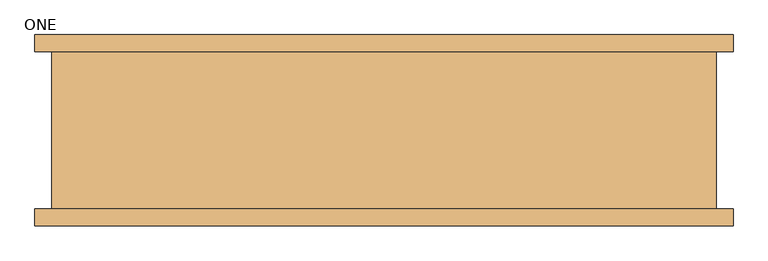
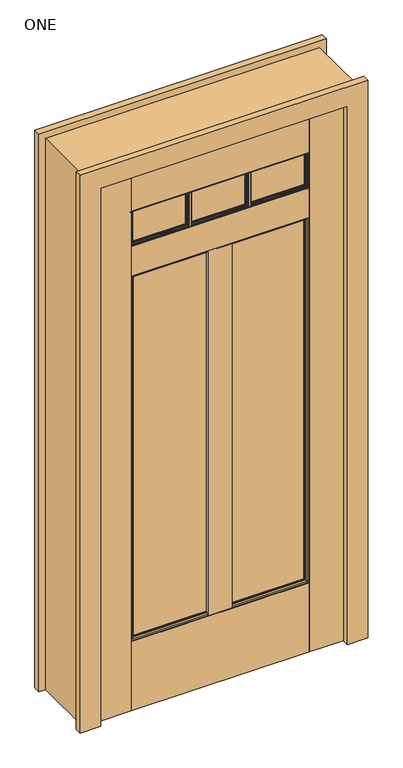
"""IFC4 building model written with IfcOpenShell, lengths in millimetres: door geometry, Door-Exterior-Simpson-Craftsman : ONE."""

import ifcopenshell
import ifcopenshell.guid

model = None  # the IFC model being written
_history = None  # IfcOwnerHistory: only IFC2X3 demands one
_inside = {}  # id of a spatial element -> (the spatial element, [elements in it])
_under = {}  # id of a project, library or spatial element -> (it, [spatial elements below it])
_declared = {}  # id of a project -> (the project, [libraries it declares])
_typed = {}  # id of a type object -> (the type object, [elements of that type])
_made_of = {}  # id of a material, layer set ... -> (it, [elements and type objects made of it])


def new_model(schema):
    """Start an empty IFC model of exactly this schema.

    Asked for "IFC4X3", IfcOpenShell would pick the latest addendum, in which some entities
    have other attributes; the version numbers below select the first issue.
    IFC2X3 requires an IfcOwnerHistory on every rooted entity: one is made here for all.
    """
    global model, _history
    if schema == "IFC4X3":
        model = ifcopenshell.file(schema_version=(4, 3, 0, 0))
    else:
        model = ifcopenshell.file(schema=schema)
    _inside.clear()
    _under.clear()
    _declared.clear()
    _typed.clear()
    _made_of.clear()
    _history = None
    if model.schema == "IFC2X3":
        org = make("IfcOrganization", Name="unknown")
        user = make(
            "IfcPersonAndOrganization",
            ThePerson=make("IfcPerson", FamilyName="unknown"),
            TheOrganization=org,
        )
        app = make(
            "IfcApplication",
            ApplicationDeveloper=org,
            Version="unknown",
            ApplicationFullName="unknown",
            ApplicationIdentifier="unknown",
        )
        _history = make(
            "IfcOwnerHistory",
            OwningUser=user,
            OwningApplication=app,
            ChangeAction="ADDED",
            CreationDate=0,
        )
    return model


def make(cls, **values):
    """One entity of the class cls with the attributes given. An attribute that is None is left unset."""
    return model.create_entity(
        cls, **{name: value for name, value in values.items() if value is not None}
    )


def rooted(cls, **values):
    """An entity with a GlobalId (a new one), such as an element, a storey or a relation."""
    return make(cls, GlobalId=ifcopenshell.guid.new(), OwnerHistory=_history, **values)


def si_unit(unit_type, name, prefix=None):
    """IfcSIUnit, for example si_unit("LENGTHUNIT", "METRE", prefix="MILLI")."""
    return make("IfcSIUnit", UnitType=unit_type, Prefix=prefix, Name=name)


def assignment(units):
    """IfcUnitAssignment: the units of a project."""
    return None if units is None else make("IfcUnitAssignment", Units=units)


def point(xyz):
    """IfcCartesianPoint."""
    return None if xyz is None else make("IfcCartesianPoint", Coordinates=xyz)


def direction(xyz):
    """IfcDirection."""
    return None if xyz is None else make("IfcDirection", DirectionRatios=xyz)


def frame(location, z_axis=None, x_axis=None):
    """IfcAxis2Placement3D, a coordinate frame: its origin and axes. An axis left out is left unset."""
    return make(
        "IfcAxis2Placement3D",
        Location=point(location),
        Axis=direction(z_axis),
        RefDirection=direction(x_axis),
    )


def frame_2d(location, x_axis=None):
    """IfcAxis2Placement2D, a coordinate frame in the plane: its origin and x axis."""
    return make(
        "IfcAxis2Placement2D", Location=point(location), RefDirection=direction(x_axis)
    )


def origin():
    """The frame at (0, 0, 0) with its axes left unset."""
    return frame((0.0, 0.0, 0.0))


def origin_with_axes():
    """The frame at (0, 0, 0) with the z axis (0, 0, 1) and the x axis (1, 0, 0) written out."""
    return frame((0.0, 0.0, 0.0), z_axis=(0.0, 0.0, 1.0), x_axis=(1.0, 0.0, 0.0))


def place(relative_to, where):
    """IfcLocalPlacement: puts the frame where relative to a parent placement (None: the world)."""
    return make(
        "IfcLocalPlacement", PlacementRelTo=relative_to, RelativePlacement=where
    )


def context(
    kind, dimensions, precision=None, world=None, true_north=None, identifier=None
):
    """IfcGeometricRepresentationContext, for example the 3D "Model" context."""
    return make(
        "IfcGeometricRepresentationContext",
        ContextIdentifier=identifier,
        ContextType=kind,
        CoordinateSpaceDimension=dimensions,
        Precision=precision,
        WorldCoordinateSystem=world,
        TrueNorth=true_north,
    )


def project(units=None, contexts=None):
    """IfcProject with its units and contexts."""
    return rooted(
        "IfcProject",
        Name="project",
        RepresentationContexts=contexts,
        UnitsInContext=assignment(units),
    )


def spatial(cls, under=None, at=None, **own):
    """A site, building, storey or space (cls), placed at a placement, below another one or the project."""
    s = rooted(cls, ObjectPlacement=at, **own)
    if under is not None:
        _under.setdefault(under.id(), (under, []))[1].append(s)
    return s


def polyline(points):
    """IfcPolyline through the points."""
    return make("IfcPolyline", Points=[point(p) for p in points])


def circle_curve(where, radius):
    """IfcCircle in the frame where."""
    return make("IfcCircle", Position=where, Radius=radius)


def ellipse_curve(where, semi_axis1, semi_axis2):
    """IfcEllipse in the frame where."""
    return make(
        "IfcEllipse", Position=where, SemiAxis1=semi_axis1, SemiAxis2=semi_axis2
    )


def trimmed(basis, trim1, trim2, sense, master):
    """IfcTrimmedCurve: the piece of a basis curve between two trims."""
    return make(
        "IfcTrimmedCurve",
        BasisCurve=basis,
        Trim1=trim1,
        Trim2=trim2,
        SenseAgreement=sense,
        MasterRepresentation=master,
    )


def segment(curve, same_sense, transition):
    """IfcCompositeCurveSegment."""
    return make(
        "IfcCompositeCurveSegment",
        Transition=transition,
        SameSense=same_sense,
        ParentCurve=curve,
    )


def composite_curve(segments, self_intersect=None):
    """IfcCompositeCurve: segments joined end to end."""
    return make("IfcCompositeCurve", Segments=segments, SelfIntersect=self_intersect)


def outline(outer, holes=None, kind="AREA"):
    """IfcArbitraryClosedProfileDef: a profile drawn as a closed curve; with holes, ...WithVoids."""
    if holes is None:
        return make("IfcArbitraryClosedProfileDef", ProfileType=kind, OuterCurve=outer)
    return make(
        "IfcArbitraryProfileDefWithVoids",
        ProfileType=kind,
        OuterCurve=outer,
        InnerCurves=holes,
    )


def extrude(swept, where, along, depth):
    """IfcExtrudedAreaSolid: the profile swept, set in the frame where, extruded along a direction by depth."""
    return make(
        "IfcExtrudedAreaSolid",
        SweptArea=swept,
        Position=where,
        ExtrudedDirection=direction(along),
        Depth=depth,
    )


def faces_of(points, faces, orient=None, outer=None):
    """IfcFace entities. A face is a list of loops; a loop is a list of indices into points, from 0.

    orient and outer hold one flag for each loop. By default every Orientation is true, the
    first loop of a face is its IfcFaceOuterBound and the others are IfcFaceBound.
    """
    made = []
    for i, loops in enumerate(faces):
        bounds = []
        for j, loop in enumerate(loops):
            is_outer = j == 0 if outer is None else outer[i][j]
            bounds.append(
                make(
                    "IfcFaceOuterBound" if is_outer else "IfcFaceBound",
                    Bound=make("IfcPolyLoop", Polygon=[points[k] for k in loop]),
                    Orientation=True if orient is None else orient[i][j],
                )
            )
        made.append(make("IfcFace", Bounds=bounds))
    return made


def faceted_brep(points, faces, orient=None, outer=None, voids=None):
    """IfcFacetedBrep: a solid bounded by flat faces; with voids (closed shells), ...WithVoids."""
    shared = [point(p) for p in points]
    hull = make("IfcClosedShell", CfsFaces=faces_of(shared, faces, orient, outer))
    if voids is None:
        return make("IfcFacetedBrep", Outer=hull)
    return make(
        "IfcFacetedBrepWithVoids",
        Outer=hull,
        Voids=[
            make(cls, CfsFaces=faces_of(shared, fs, o, b)) for cls, fs, o, b in voids
        ],
    )


def shape(context_of_items, identifier, shape_type, items):
    """IfcShapeRepresentation: the items that make up one representation, for example the "Body"."""
    return make(
        "IfcShapeRepresentation",
        ContextOfItems=context_of_items,
        RepresentationIdentifier=identifier,
        RepresentationType=shape_type,
        Items=items,
    )


def source(mapping_origin, context_of_items, identifier, shape_type, items):
    """IfcRepresentationMap: a shape defined once, which mapped items show again and again."""
    return make(
        "IfcRepresentationMap",
        MappingOrigin=mapping_origin,
        MappedRepresentation=shape(context_of_items, identifier, shape_type, items),
    )


def transform(
    local_origin,
    x_axis=None,
    y_axis=None,
    z_axis=None,
    scale=None,
    scale2=None,
    scale3=None,
    uniform=True,
):
    """IfcCartesianTransformationOperator3D, or its non-uniform kind. x_axis, y_axis, z_axis: its Axis1, 2, 3."""
    if uniform:
        return make(
            "IfcCartesianTransformationOperator3D",
            Axis1=direction(x_axis),
            Axis2=direction(y_axis),
            LocalOrigin=point(local_origin),
            Scale=scale,
            Axis3=direction(z_axis),
        )
    return make(
        "IfcCartesianTransformationOperator3DnonUniform",
        Axis1=direction(x_axis),
        Axis2=direction(y_axis),
        LocalOrigin=point(local_origin),
        Scale=scale,
        Axis3=direction(z_axis),
        Scale2=scale2,
        Scale3=scale3,
    )


def mapped(mapping_source, mapping_target):
    """IfcMappedItem: shows the shape of a source again, moved by a transform."""
    return make(
        "IfcMappedItem", MappingSource=mapping_source, MappingTarget=mapping_target
    )


def made_of(thing, what):
    """Note that an element or type object is made of a material, layer set ...; save() writes the relation."""
    if what is not None:
        _made_of.setdefault(what.id(), (what, []))[1].append(thing)
    return thing


def element(
    cls,
    number,
    at=None,
    inside=None,
    cuts=None,
    type_object=None,
    material=None,
    context=None,
    identifier="Body",
    shape_type=None,
    held_by="IfcProductDefinitionShape",
    body=None,
    shapes=None,
    **own,
):
    """One element of the class cls, such as IfcWall. Its Tag is "e" and its number.

    at: its placement. inside: the storey or other place that contains it. cuts: it is an
    opening in that element (IfcRelVoidsElement). A single representation is given by context,
    identifier, shape_type and body (its items); several are given by shapes. held_by: the class
    of the entity that holds the representations. save() writes the other relations.
    """
    e = rooted(cls, Tag="e%d" % number, ObjectPlacement=at, **own)
    if body is not None:
        shapes = [shape(context, identifier, shape_type, body)]
    if shapes is not None:
        e.Representation = make(held_by, Representations=shapes)
    if inside is not None:
        _inside.setdefault(inside.id(), (inside, []))[1].append(e)
    if cuts is not None:
        rooted(
            "IfcRelVoidsElement", RelatingBuildingElement=cuts, RelatedOpeningElement=e
        )
    if type_object is not None:
        _typed.setdefault(type_object.id(), (type_object, []))[1].append(e)
    return made_of(e, material)


def aggregate(whole, parts):
    """IfcRelAggregates: a whole, such as a stair, and the parts it consists of."""
    return rooted("IfcRelAggregates", RelatingObject=whole, RelatedObjects=parts)


def save(model, path):
    """Write the relations noted so far, then the file.

    IfcRelAggregates (storeys below a building ...), IfcRelContainedInSpatialStructure (elements
    in a storey), IfcRelDefinesByType, IfcRelAssociatesMaterial and IfcRelDeclares: one each for
    every whole, place, type object, material and project.
    """
    for whole, parts in _under.values():
        aggregate(whole, parts)
    for where, things in _inside.values():
        rooted(
            "IfcRelContainedInSpatialStructure",
            RelatedElements=things,
            RelatingStructure=where,
        )
    for kind, things in _typed.values():
        rooted("IfcRelDefinesByType", RelatedObjects=things, RelatingType=kind)
    for what, things in _made_of.values():
        rooted("IfcRelAssociatesMaterial", RelatedObjects=things, RelatingMaterial=what)
    for by, libraries in _declared.values():
        rooted("IfcRelDeclares", RelatingContext=by, RelatedDefinitions=libraries)
    model.write(path)


def plane_surface(at):
    """IfcPlane: the flat surface through the origin of the frame at, square to its z axis."""
    return make("IfcPlane", Position=at)


def cylinder_surface(at, radius):
    """IfcCylindricalSurface: all points at the distance radius from the z axis of the frame at."""
    return make("IfcCylindricalSurface", Position=at, Radius=radius)


def advanced_brep(points, edges, surfaces, faces):
    """IfcAdvancedBrep: a solid bounded by faces that lie on surfaces and meet in shared edges.

    An edge is (start, end): straight between two places in points (the first is 0);
    or (start, end, curve); or (start, end, curve, False) where it runs against its curve.
    A face is (place in surfaces, loops), or (place, loops, False) where it looks against
    its surface's normal. A loop lists edges by number (the first is 1), with a minus sign
    where the edge is run from its end to its start. The first loop is the outer one.
    """
    corners = [point(p) for p in points]
    vertices = [make("IfcVertexPoint", VertexGeometry=c) for c in corners]
    made = []
    for start, end, *more in edges:
        made.append(
            make(
                "IfcEdgeCurve",
                EdgeStart=vertices[start],
                EdgeEnd=vertices[end],
                EdgeGeometry=more[0] if more else make("IfcPolyline", Points=[corners[start], corners[end]]),
                SameSense=more[1] if len(more) > 1 else True,
            )
        )
    hull = []
    for where, loops, *sense in faces:
        bounds = []
        for j, loop in enumerate(loops):
            ring = [make("IfcOrientedEdge", EdgeElement=made[abs(k) - 1], Orientation=k > 0) for k in loop]
            bounds.append(
                make(
                    "IfcFaceOuterBound" if j == 0 else "IfcFaceBound",
                    Bound=make("IfcEdgeLoop", EdgeList=ring),
                    Orientation=True,
                )
            )
        hull.append(make("IfcAdvancedFace", Bounds=bounds, FaceSurface=surfaces[where], SameSense=sense[0] if sense else True))
    return make("IfcAdvancedBrep", Outer=make("IfcClosedShell", CfsFaces=hull))


def one_efa2d6c3(model_context):
    return source(origin(), model_context, "Body", "SolidModel", [
        extrude(outline(composite_curve([segment(polyline([(114.0354167, -78.5495), (114.0354167, -80.264), (116.1486027, -80.6366117)]), True, "CONTINUOUS"), segment(trimmed(circle_curve(frame_2d((115.7075363, -83.1380234)), 2.54), [point((116.1486027, -80.6366117))], [point((118.208948, -82.696957))], False, "CARTESIAN"), True, "CONTINUOUS"), segment(polyline([(118.208948, -82.696957), (118.7696182, -85.8766758), (120.0821906, -85.991511)]), True, "CONTINUOUS"), segment(trimmed(circle_curve(frame_2d((120.0157779, -86.7506113)), 0.762), [point((120.0821906, -85.991511))], [point((120.7662014, -86.6182914))], False, "CARTESIAN"), True, "CONTINUOUS"), segment(polyline([(120.7662014, -86.6182914), (121.1685282, -88.9), (98.9648051, -88.9), (99.3671319, -86.6182914)]), True, "CONTINUOUS"), segment(trimmed(circle_curve(frame_2d((100.1175554, -86.7506113)), 0.762), [point((99.3671319, -86.6182914))], [point((100.0511427, -85.991511))], False, "CARTESIAN"), True, "CONTINUOUS"), segment(polyline([(100.0511427, -85.991511), (101.3637152, -85.8766758), (101.9243854, -82.696957)]), True, "CONTINUOUS"), segment(trimmed(circle_curve(frame_2d((104.4257971, -83.1380234)), 2.54), [point((101.9243854, -82.696957))], [point((103.9847307, -80.6366117))], False, "CARTESIAN"), True, "CONTINUOUS"), segment(polyline([(103.9847307, -80.6366117), (106.0979167, -80.264), (106.0979167, -78.5495), (114.0354167, -78.5495)]), True, "CONTINUOUS")], self_intersect=False)), frame((0.0, 0.0, 1817.6875), z_axis=(0.0, 0.0, 1.0), x_axis=(1.0, 0.0, 0.0)), (0.0, 0.0, 1.0), 139.7),
        extrude(outline(composite_curve([segment(polyline([(114.0354167, -118.3005), (106.0979167, -118.3005), (106.0979167, -116.586), (103.9847307, -116.2133883)]), True, "CONTINUOUS"), segment(trimmed(circle_curve(frame_2d((104.4257971, -113.7119766)), 2.54), [point((103.9847307, -116.2133883))], [point((101.9243854, -114.153043))], False, "CARTESIAN"), True, "CONTINUOUS"), segment(polyline([(101.9243854, -114.153043), (101.3637152, -110.9733242), (100.0511427, -110.858489)]), True, "CONTINUOUS"), segment(trimmed(circle_curve(frame_2d((100.1175554, -110.0993887)), 0.762), [point((100.0511427, -110.858489))], [point((99.3671319, -110.2317086))], False, "CARTESIAN"), True, "CONTINUOUS"), segment(polyline([(99.3671319, -110.2317086), (98.9648051, -107.95), (121.1685282, -107.95), (120.7662014, -110.2317086)]), True, "CONTINUOUS"), segment(trimmed(circle_curve(frame_2d((120.0157779, -110.0993887)), 0.762), [point((120.7662014, -110.2317086))], [point((120.0821906, -110.858489))], False, "CARTESIAN"), True, "CONTINUOUS"), segment(polyline([(120.0821906, -110.858489), (118.7696182, -110.9733242), (118.208948, -114.153043)]), True, "CONTINUOUS"), segment(trimmed(circle_curve(frame_2d((115.7075363, -113.7119766)), 2.54), [point((118.208948, -114.153043))], [point((116.1486027, -116.2133883))], False, "CARTESIAN"), True, "CONTINUOUS"), segment(polyline([(116.1486027, -116.2133883), (114.0354167, -116.586), (114.0354167, -118.3005)]), True, "CONTINUOUS")], self_intersect=False)), frame((0.0, 0.0, 1817.6875), z_axis=(0.0, 0.0, 1.0), x_axis=(1.0, 0.0, 0.0)), (0.0, 0.0, 1.0), 139.7),
        extrude(outline(composite_curve([segment(polyline([(-106.0979167, -78.5495), (-106.0979167, -80.264), (-103.9847307, -80.6366117)]), True, "CONTINUOUS"), segment(trimmed(circle_curve(frame_2d((-104.4257971, -83.1380234)), 2.54), [point((-103.9847307, -80.6366117))], [point((-101.9243854, -82.696957))], False, "CARTESIAN"), True, "CONTINUOUS"), segment(polyline([(-101.9243854, -82.696957), (-101.3637152, -85.8766758), (-100.0511427, -85.991511)]), True, "CONTINUOUS"), segment(trimmed(circle_curve(frame_2d((-100.1175554, -86.7506113)), 0.762), [point((-100.0511427, -85.991511))], [point((-99.3671319, -86.6182914))], False, "CARTESIAN"), True, "CONTINUOUS"), segment(polyline([(-99.3671319, -86.6182914), (-98.9648051, -88.9), (-121.1685282, -88.9), (-120.7662014, -86.6182914)]), True, "CONTINUOUS"), segment(trimmed(circle_curve(frame_2d((-120.0157779, -86.7506113)), 0.762), [point((-120.7662014, -86.6182914))], [point((-120.0821906, -85.991511))], False, "CARTESIAN"), True, "CONTINUOUS"), segment(polyline([(-120.0821906, -85.991511), (-118.7696182, -85.8766758), (-118.208948, -82.696957)]), True, "CONTINUOUS"), segment(trimmed(circle_curve(frame_2d((-115.7075363, -83.1380234)), 2.54), [point((-118.208948, -82.696957))], [point((-116.1486027, -80.6366117))], False, "CARTESIAN"), True, "CONTINUOUS"), segment(polyline([(-116.1486027, -80.6366117), (-114.0354167, -80.264), (-114.0354167, -78.5495), (-106.0979167, -78.5495)]), True, "CONTINUOUS")], self_intersect=False)), frame((0.0, 0.0, 1817.6875), z_axis=(0.0, 0.0, 1.0), x_axis=(1.0, 0.0, 0.0)), (0.0, 0.0, 1.0), 139.7),
        extrude(outline(composite_curve([segment(polyline([(-106.0979167, -118.3005), (-114.0354167, -118.3005), (-114.0354167, -116.586), (-116.1486027, -116.2133883)]), True, "CONTINUOUS"), segment(trimmed(circle_curve(frame_2d((-115.7075363, -113.7119766)), 2.54), [point((-116.1486027, -116.2133883))], [point((-118.208948, -114.153043))], False, "CARTESIAN"), True, "CONTINUOUS"), segment(polyline([(-118.208948, -114.153043), (-118.7696182, -110.9733242), (-120.0821906, -110.858489)]), True, "CONTINUOUS"), segment(trimmed(circle_curve(frame_2d((-120.0157779, -110.0993887)), 0.762), [point((-120.0821906, -110.858489))], [point((-120.7662014, -110.2317086))], False, "CARTESIAN"), True, "CONTINUOUS"), segment(polyline([(-120.7662014, -110.2317086), (-121.1685282, -107.95), (-98.9648051, -107.95), (-99.3671319, -110.2317086)]), True, "CONTINUOUS"), segment(trimmed(circle_curve(frame_2d((-100.1175554, -110.0993887)), 0.762), [point((-99.3671319, -110.2317086))], [point((-100.0511427, -110.858489))], False, "CARTESIAN"), True, "CONTINUOUS"), segment(polyline([(-100.0511427, -110.858489), (-101.3637152, -110.9733242), (-101.9243854, -114.153043)]), True, "CONTINUOUS"), segment(trimmed(circle_curve(frame_2d((-104.4257971, -113.7119766)), 2.54), [point((-101.9243854, -114.153043))], [point((-103.9847307, -116.2133883))], False, "CARTESIAN"), True, "CONTINUOUS"), segment(polyline([(-103.9847307, -116.2133883), (-106.0979167, -116.586), (-106.0979167, -118.3005)]), True, "CONTINUOUS")], self_intersect=False)), frame((0.0, 0.0, 1817.6875), z_axis=(0.0, 0.0, 1.0), x_axis=(1.0, 0.0, 0.0)), (0.0, 0.0, 1.0), 139.7),
        extrude(outline(polyline([(44.45, -78.7796875), (44.45, -118.0703125), (-44.45, -118.0703125), (-44.45, -78.7796875), (44.45, -78.7796875)])), frame((0.0, 0.0, 271.4625), z_axis=(0.0, 0.0, 1.0), x_axis=(1.0, 0.0, 0.0)), (0.0, 0.0, 1.0), 1431.925),
        extrude(outline(polyline([(419.89375, -78.7796875), (419.89375, -118.0703125), (330.99375, -118.0703125), (330.99375, -78.7796875), (419.89375, -78.7796875)])), frame((0.0, 0.0, 271.4625), z_axis=(0.0, 0.0, 1.0), x_axis=(1.0, 0.0, 0.0)), (0.0, 0.0, 1.0), 1431.925),
        extrude(outline(polyline([(-330.99375, -78.7796875), (-330.99375, -118.0703125), (-419.89375, -118.0703125), (-419.89375, -78.7796875), (-330.99375, -78.7796875)])), frame((0.0, 0.0, 271.4625), z_axis=(0.0, 0.0, 1.0), x_axis=(1.0, 0.0, 0.0)), (0.0, 0.0, 1.0), 1431.925),
        extrude(outline(polyline([(330.2, -107.95), (-330.2, -107.95), (-330.2, -88.9), (330.2, -88.9), (330.2, -107.95)])), frame((0.0, 0.0, 271.4625), z_axis=(0.0, 0.0, 1.0), x_axis=(1.0, 0.0, 0.0)), (0.0, 0.0, 1.0), 1431.925),
        extrude(outline(composite_curve([segment(polyline([(334.16875, -78.5495), (334.16875, -80.264), (336.281936, -80.6366117)]), True, "CONTINUOUS"), segment(trimmed(circle_curve(frame_2d((335.8408696, -83.1380234)), 2.54), [point((336.281936, -80.6366117))], [point((338.3422813, -82.696957))], False, "CARTESIAN"), True, "CONTINUOUS"), segment(polyline([(338.3422813, -82.696957), (338.9029515, -85.8766758), (340.2155239, -85.991511)]), True, "CONTINUOUS"), segment(trimmed(circle_curve(frame_2d((340.1491113, -86.7506113)), 0.762), [point((340.2155239, -85.991511))], [point((340.8995348, -86.6182914))], False, "CARTESIAN"), True, "CONTINUOUS"), segment(polyline([(340.8995348, -86.6182914), (341.3018616, -88.9), (319.0981384, -88.9), (319.5004652, -86.6182914)]), True, "CONTINUOUS"), segment(trimmed(circle_curve(frame_2d((320.2508887, -86.7506113)), 0.762), [point((319.5004652, -86.6182914))], [point((320.1844761, -85.991511))], False, "CARTESIAN"), True, "CONTINUOUS"), segment(polyline([(320.1844761, -85.991511), (321.4970485, -85.8766758), (322.0577187, -82.696957)]), True, "CONTINUOUS"), segment(trimmed(circle_curve(frame_2d((324.5591304, -83.1380234)), 2.54), [point((322.0577187, -82.696957))], [point((324.118064, -80.6366117))], False, "CARTESIAN"), True, "CONTINUOUS"), segment(polyline([(324.118064, -80.6366117), (326.23125, -80.264), (326.23125, -78.5495), (334.16875, -78.5495)]), True, "CONTINUOUS")], self_intersect=False)), frame((0.0, 0.0, 1817.6875), z_axis=(0.0, 0.0, 1.0), x_axis=(1.0, 0.0, 0.0)), (0.0, 0.0, 1.0), 139.7),
        extrude(outline(composite_curve([segment(polyline([(334.16875, -118.3005), (326.23125, -118.3005), (326.23125, -116.586), (324.118064, -116.2133883)]), True, "CONTINUOUS"), segment(trimmed(circle_curve(frame_2d((324.5591304, -113.7119766)), 2.54), [point((324.118064, -116.2133883))], [point((322.0577187, -114.153043))], False, "CARTESIAN"), True, "CONTINUOUS"), segment(polyline([(322.0577187, -114.153043), (321.4970485, -110.9733242), (320.1844761, -110.858489)]), True, "CONTINUOUS"), segment(trimmed(circle_curve(frame_2d((320.2508887, -110.0993887)), 0.762), [point((320.1844761, -110.858489))], [point((319.5004652, -110.2317086))], False, "CARTESIAN"), True, "CONTINUOUS"), segment(polyline([(319.5004652, -110.2317086), (319.0981384, -107.95), (341.3018616, -107.95), (340.8995348, -110.2317086)]), True, "CONTINUOUS"), segment(trimmed(circle_curve(frame_2d((340.1491113, -110.0993887)), 0.762), [point((340.8995348, -110.2317086))], [point((340.2155239, -110.858489))], False, "CARTESIAN"), True, "CONTINUOUS"), segment(polyline([(340.2155239, -110.858489), (338.9029515, -110.9733242), (338.3422813, -114.153043)]), True, "CONTINUOUS"), segment(trimmed(circle_curve(frame_2d((335.8408696, -113.7119766)), 2.54), [point((338.3422813, -114.153043))], [point((336.281936, -116.2133883))], False, "CARTESIAN"), True, "CONTINUOUS"), segment(polyline([(336.281936, -116.2133883), (334.16875, -116.586), (334.16875, -118.3005)]), True, "CONTINUOUS")], self_intersect=False)), frame((0.0, 0.0, 1817.6875), z_axis=(0.0, 0.0, 1.0), x_axis=(1.0, 0.0, 0.0)), (0.0, 0.0, 1.0), 139.7),
        extrude(outline(composite_curve([segment(polyline([(-78.5495, 1813.71875), (-80.264, 1813.71875), (-80.6366117, 1811.605564)]), True, "CONTINUOUS"), segment(trimmed(circle_curve(frame_2d((-83.1380234, 1812.0466304)), 2.54), [point((-80.6366117, 1811.605564))], [point((-82.696957, 1809.5452187))], False, "CARTESIAN"), True, "CONTINUOUS"), segment(polyline([(-82.696957, 1809.5452187), (-85.8766758, 1808.9845485), (-85.991511, 1807.6719761)]), True, "CONTINUOUS"), segment(trimmed(circle_curve(frame_2d((-86.7506113, 1807.7383887)), 0.762), [point((-85.991511, 1807.6719761))], [point((-86.6182914, 1806.9879652))], False, "CARTESIAN"), True, "CONTINUOUS"), segment(polyline([(-86.6182914, 1806.9879652), (-88.9, 1806.5856384), (-88.9, 1828.7893616), (-86.6182914, 1828.3870348)]), True, "CONTINUOUS"), segment(trimmed(circle_curve(frame_2d((-86.7506113, 1827.6366113)), 0.762), [point((-86.6182914, 1828.3870348))], [point((-85.991511, 1827.7030239))], False, "CARTESIAN"), True, "CONTINUOUS"), segment(polyline([(-85.991511, 1827.7030239), (-85.8766758, 1826.3904515), (-82.696957, 1825.8297813)]), True, "CONTINUOUS"), segment(trimmed(circle_curve(frame_2d((-83.1380234, 1823.3283696)), 2.54), [point((-82.696957, 1825.8297813))], [point((-80.6366117, 1823.769436))], False, "CARTESIAN"), True, "CONTINUOUS"), segment(polyline([(-80.6366117, 1823.769436), (-80.264, 1821.65625), (-78.5495, 1821.65625), (-78.5495, 1813.71875)]), True, "CONTINUOUS")], self_intersect=False)), frame((-330.2, 0.0, 0.0), z_axis=(1.0, 0.0, 0.0), x_axis=(0.0, 1.0, 0.0)), (0.0, 0.0, 1.0), 660.4),
        extrude(outline(composite_curve([segment(polyline([(-118.3005, 1813.71875), (-118.3005, 1821.65625), (-116.586, 1821.65625), (-116.2133883, 1823.769436)]), True, "CONTINUOUS"), segment(trimmed(circle_curve(frame_2d((-113.7119766, 1823.3283696)), 2.54), [point((-116.2133883, 1823.769436))], [point((-114.153043, 1825.8297813))], False, "CARTESIAN"), True, "CONTINUOUS"), segment(polyline([(-114.153043, 1825.8297813), (-110.9733242, 1826.3904515), (-110.858489, 1827.7030239)]), True, "CONTINUOUS"), segment(trimmed(circle_curve(frame_2d((-110.0993887, 1827.6366113)), 0.762), [point((-110.858489, 1827.7030239))], [point((-110.2317086, 1828.3870348))], False, "CARTESIAN"), True, "CONTINUOUS"), segment(polyline([(-110.2317086, 1828.3870348), (-107.95, 1828.7893616), (-107.95, 1806.5856384), (-110.2317086, 1806.9879652)]), True, "CONTINUOUS"), segment(trimmed(circle_curve(frame_2d((-110.0993887, 1807.7383887)), 0.762), [point((-110.2317086, 1806.9879652))], [point((-110.858489, 1807.6719761))], False, "CARTESIAN"), True, "CONTINUOUS"), segment(polyline([(-110.858489, 1807.6719761), (-110.9733242, 1808.9845485), (-114.153043, 1809.5452187)]), True, "CONTINUOUS"), segment(trimmed(circle_curve(frame_2d((-113.7119766, 1812.0466304)), 2.54), [point((-114.153043, 1809.5452187))], [point((-116.2133883, 1811.605564))], False, "CARTESIAN"), True, "CONTINUOUS"), segment(polyline([(-116.2133883, 1811.605564), (-116.586, 1813.71875), (-118.3005, 1813.71875)]), True, "CONTINUOUS")], self_intersect=False)), frame((-330.2, 0.0, 0.0), z_axis=(1.0, 0.0, 0.0), x_axis=(0.0, 1.0, 0.0)), (0.0, 0.0, 1.0), 660.4),
        extrude(outline(composite_curve([segment(polyline([(-78.5495, 1953.41875), (-80.264, 1953.41875), (-80.6366117, 1951.305564)]), True, "CONTINUOUS"), segment(trimmed(circle_curve(frame_2d((-83.1380234, 1951.7466304)), 2.54), [point((-80.6366117, 1951.305564))], [point((-82.696957, 1949.2452187))], False, "CARTESIAN"), True, "CONTINUOUS"), segment(polyline([(-82.696957, 1949.2452187), (-85.8766758, 1948.6845485), (-85.991511, 1947.3719761)]), True, "CONTINUOUS"), segment(trimmed(circle_curve(frame_2d((-86.7506113, 1947.4383887)), 0.762), [point((-85.991511, 1947.3719761))], [point((-86.6182914, 1946.6879652))], False, "CARTESIAN"), True, "CONTINUOUS"), segment(polyline([(-86.6182914, 1946.6879652), (-88.9, 1946.2856384), (-88.9, 1968.4893616), (-86.6182914, 1968.0870348)]), True, "CONTINUOUS"), segment(trimmed(circle_curve(frame_2d((-86.7506113, 1967.3366113)), 0.762), [point((-86.6182914, 1968.0870348))], [point((-85.991511, 1967.4030239))], False, "CARTESIAN"), True, "CONTINUOUS"), segment(polyline([(-85.991511, 1967.4030239), (-85.8766758, 1966.0904515), (-82.696957, 1965.5297813)]), True, "CONTINUOUS"), segment(trimmed(circle_curve(frame_2d((-83.1380234, 1963.0283696)), 2.54), [point((-82.696957, 1965.5297813))], [point((-80.6366117, 1963.469436))], False, "CARTESIAN"), True, "CONTINUOUS"), segment(polyline([(-80.6366117, 1963.469436), (-80.264, 1961.35625), (-78.5495, 1961.35625), (-78.5495, 1953.41875)]), True, "CONTINUOUS")], self_intersect=False)), frame((-330.2, 0.0, 0.0), z_axis=(1.0, 0.0, 0.0), x_axis=(0.0, 1.0, 0.0)), (0.0, 0.0, 1.0), 660.4),
        extrude(outline(composite_curve([segment(polyline([(-118.3005, 1953.41875), (-118.3005, 1961.35625), (-116.586, 1961.35625), (-116.2133883, 1963.469436)]), True, "CONTINUOUS"), segment(trimmed(circle_curve(frame_2d((-113.7119766, 1963.0283696)), 2.54), [point((-116.2133883, 1963.469436))], [point((-114.153043, 1965.5297813))], False, "CARTESIAN"), True, "CONTINUOUS"), segment(polyline([(-114.153043, 1965.5297813), (-110.9733242, 1966.0904515), (-110.858489, 1967.4030239)]), True, "CONTINUOUS"), segment(trimmed(circle_curve(frame_2d((-110.0993887, 1967.3366113)), 0.762), [point((-110.858489, 1967.4030239))], [point((-110.2317086, 1968.0870348))], False, "CARTESIAN"), True, "CONTINUOUS"), segment(polyline([(-110.2317086, 1968.0870348), (-107.95, 1968.4893616), (-107.95, 1946.2856384), (-110.2317086, 1946.6879652)]), True, "CONTINUOUS"), segment(trimmed(circle_curve(frame_2d((-110.0993887, 1947.4383887)), 0.762), [point((-110.2317086, 1946.6879652))], [point((-110.858489, 1947.3719761))], False, "CARTESIAN"), True, "CONTINUOUS"), segment(polyline([(-110.858489, 1947.3719761), (-110.9733242, 1948.6845485), (-114.153043, 1949.2452187)]), True, "CONTINUOUS"), segment(trimmed(circle_curve(frame_2d((-113.7119766, 1951.7466304)), 2.54), [point((-114.153043, 1949.2452187))], [point((-116.2133883, 1951.305564))], False, "CARTESIAN"), True, "CONTINUOUS"), segment(polyline([(-116.2133883, 1951.305564), (-116.586, 1953.41875), (-118.3005, 1953.41875)]), True, "CONTINUOUS")], self_intersect=False)), frame((-330.2, 0.0, 0.0), z_axis=(1.0, 0.0, 0.0), x_axis=(0.0, 1.0, 0.0)), (0.0, 0.0, 1.0), 660.4),
        extrude(outline(composite_curve([segment(polyline([(-326.23125, -78.5495), (-326.23125, -80.264), (-324.118064, -80.6366117)]), True, "CONTINUOUS"), segment(trimmed(circle_curve(frame_2d((-324.5591304, -83.1380234)), 2.54), [point((-324.118064, -80.6366117))], [point((-322.0577187, -82.696957))], False, "CARTESIAN"), True, "CONTINUOUS"), segment(polyline([(-322.0577187, -82.696957), (-321.4970485, -85.8766758), (-320.1844761, -85.991511)]), True, "CONTINUOUS"), segment(trimmed(circle_curve(frame_2d((-320.2508887, -86.7506113)), 0.762), [point((-320.1844761, -85.991511))], [point((-319.5004652, -86.6182914))], False, "CARTESIAN"), True, "CONTINUOUS"), segment(polyline([(-319.5004652, -86.6182914), (-319.0981384, -88.9), (-341.3018616, -88.9), (-340.8995348, -86.6182914)]), True, "CONTINUOUS"), segment(trimmed(circle_curve(frame_2d((-340.1491113, -86.7506113)), 0.762), [point((-340.8995348, -86.6182914))], [point((-340.2155239, -85.991511))], False, "CARTESIAN"), True, "CONTINUOUS"), segment(polyline([(-340.2155239, -85.991511), (-338.9029515, -85.8766758), (-338.3422813, -82.696957)]), True, "CONTINUOUS"), segment(trimmed(circle_curve(frame_2d((-335.8408696, -83.1380234)), 2.54), [point((-338.3422813, -82.696957))], [point((-336.281936, -80.6366117))], False, "CARTESIAN"), True, "CONTINUOUS"), segment(polyline([(-336.281936, -80.6366117), (-334.16875, -80.264), (-334.16875, -78.5495), (-326.23125, -78.5495)]), True, "CONTINUOUS")], self_intersect=False)), frame((0.0, 0.0, 1817.6875), z_axis=(0.0, 0.0, 1.0), x_axis=(1.0, 0.0, 0.0)), (0.0, 0.0, 1.0), 139.7),
        extrude(outline(composite_curve([segment(polyline([(-326.23125, -118.3005), (-334.16875, -118.3005), (-334.16875, -116.586), (-336.281936, -116.2133883)]), True, "CONTINUOUS"), segment(trimmed(circle_curve(frame_2d((-335.8408696, -113.7119766)), 2.54), [point((-336.281936, -116.2133883))], [point((-338.3422813, -114.153043))], False, "CARTESIAN"), True, "CONTINUOUS"), segment(polyline([(-338.3422813, -114.153043), (-338.9029515, -110.9733242), (-340.2155239, -110.858489)]), True, "CONTINUOUS"), segment(trimmed(circle_curve(frame_2d((-340.1491113, -110.0993887)), 0.762), [point((-340.2155239, -110.858489))], [point((-340.8995348, -110.2317086))], False, "CARTESIAN"), True, "CONTINUOUS"), segment(polyline([(-340.8995348, -110.2317086), (-341.3018616, -107.95), (-319.0981384, -107.95), (-319.5004652, -110.2317086)]), True, "CONTINUOUS"), segment(trimmed(circle_curve(frame_2d((-320.2508887, -110.0993887)), 0.762), [point((-319.5004652, -110.2317086))], [point((-320.1844761, -110.858489))], False, "CARTESIAN"), True, "CONTINUOUS"), segment(polyline([(-320.1844761, -110.858489), (-321.4970485, -110.9733242), (-322.0577187, -114.153043)]), True, "CONTINUOUS"), segment(trimmed(circle_curve(frame_2d((-324.5591304, -113.7119766)), 2.54), [point((-322.0577187, -114.153043))], [point((-324.118064, -116.2133883))], False, "CARTESIAN"), True, "CONTINUOUS"), segment(polyline([(-324.118064, -116.2133883), (-326.23125, -116.586), (-326.23125, -118.3005)]), True, "CONTINUOUS")], self_intersect=False)), frame((0.0, 0.0, 1817.6875), z_axis=(0.0, 0.0, 1.0), x_axis=(1.0, 0.0, 0.0)), (0.0, 0.0, 1.0), 139.7),
        extrude(outline(polyline([(-330.2, -76.2), (-330.2, -120.65), (-457.2, -120.65), (-457.2, -76.2), (-330.2, -76.2)])), origin_with_axes(), (0.0, 0.0, 1.0), 2108.2),
        extrude(outline(polyline([(457.2, -76.2), (457.2, -120.65), (330.2, -120.65), (330.2, -76.2), (457.2, -76.2)])), origin_with_axes(), (0.0, 0.0, 1.0), 2108.2),
        extrude(outline(polyline([(330.2, -88.9), (330.2, -107.95), (-330.2, -107.95), (-330.2, -88.9), (330.2, -88.9)])), frame((0.0, 0.0, 1817.6875), z_axis=(0.0, 0.0, 1.0), x_axis=(1.0, 0.0, 0.0)), (0.0, 0.0, 1.0), 139.7),
        extrude(outline(polyline([(330.2, -76.2), (330.2, -120.65), (-330.2, -120.65), (-330.2, -76.2), (330.2, -76.2)])), frame((0.0, 0.0, 1957.3875), z_axis=(0.0, 0.0, 1.0), x_axis=(1.0, 0.0, 0.0)), (0.0, 0.0, 1.0), 150.8125),
        extrude(outline(polyline([(330.2, -76.2), (330.2, -120.65), (-330.2, -120.65), (-330.2, -76.2), (330.2, -76.2)])), frame((0.0, 0.0, 1703.3875), z_axis=(0.0, 0.0, 1.0), x_axis=(1.0, 0.0, 0.0)), (0.0, 0.0, 1.0), 114.3),
        extrude(outline(polyline([(330.2, -76.2), (330.2, -120.65), (-330.2, -120.65), (-330.2, -76.2), (330.2, -76.2)])), origin_with_axes(), (0.0, 0.0, 1.0), 271.4625),
        advanced_brep(
        [(-317.7512275, -110.8215438, 283.9112725), (317.7512275, -110.8215438, 283.9112725), (317.5, -107.95, 284.1625), (-317.5, -107.95, 284.1625), (-319.4070341, -112.5663998, 282.2554659), (319.4070341, -112.5663998, 282.2554659), (-320.6823867, -112.7456389, 280.9801133), (320.6823867, -112.7456389, 280.9801133), (-324.4223446, -117.3099547, 277.2401554), (324.4223446, -117.3099547, 277.2401554), (-330.2, -118.1219512, 271.4625), (330.2, -118.1219512, 271.4625), (-330.2, -107.95, 271.4625), (330.2, -107.95, 271.4625), (317.7512275, -110.8215438, 1690.9387275), (317.5, -107.95, 1690.6875), (319.4070341, -112.5663998, 1692.5945341), (320.6823867, -112.7456389, 1693.8698867), (324.4223446, -117.3099547, 1697.6098446), (330.2, -118.1219512, 1703.3875), (330.2, -107.95, 1703.3875), (-317.7512275, -110.8215438, 1690.9387275), (-317.5, -107.95, 1690.6875), (-319.4070341, -112.5663998, 1692.5945341), (-320.6823867, -112.7456389, 1693.8698867), (-324.4223446, -117.3099547, 1697.6098446), (-330.2, -118.1219512, 1703.3875), (-330.2, -107.95, 1703.3875)],
        [
            (0, 1),
            (1, 2),
            (2, 3),
            (3, 0),
            (4, 5),
            (5, 1, ellipse_curve(frame((319.6759231, -110.6531547, 281.9865769), z_axis=(-0.7071067811865475, 0.0, -0.7071067811865475), x_axis=(-0.7071067811865476, 0.0, 0.7071067811865474)), 2.732328, 1.9320476)),
            (0, 4, ellipse_curve(frame((-319.6759231, -110.6531547, 281.9865769), z_axis=(0.7071067811865475, 0.0, -0.7071067811865475), x_axis=(-0.7071067811865476, 0.0, -0.7071067811865474)), 2.732328, 1.9320476)),
            (6, 7),
            (7, 5),
            (4, 6),
            (8, 9),
            (9, 7, ellipse_curve(frame((325.0281918, -112.9991278, 276.6343082), z_axis=(-0.7071067811865475, 0.0, -0.7071067811865475), x_axis=(-0.7071067811865476, 0.0, 0.7071067811865474)), 6.1563429, 4.3531918)),
            (6, 8, ellipse_curve(frame((-325.0281918, -112.9991278, 276.6343082), z_axis=(0.7071067811865475, 0.0, -0.7071067811865475), x_axis=(-0.7071067811865476, 0.0, -0.7071067811865474)), 6.1563429, 4.3531918)),
            (10, 11),
            (11, 9),
            (8, 10),
            (12, 13),
            (13, 11),
            (10, 12),
            (1, 14),
            (14, 15),
            (15, 2),
            (5, 16),
            (16, 14, ellipse_curve(frame((319.6759231, -110.6531547, 1692.8634231), z_axis=(0.7071067811865475, 0.0, -0.7071067811865475), x_axis=(-0.7071067811865474, 0.0, -0.7071067811865476)), 2.732328, 1.9320476)),
            (7, 17),
            (17, 16),
            (9, 18),
            (18, 17, ellipse_curve(frame((325.0281918, -112.9991278, 1698.2156918), z_axis=(0.7071067811865475, 0.0, -0.7071067811865475), x_axis=(-0.7071067811865474, 0.0, -0.7071067811865476)), 6.1563429, 4.3531918)),
            (11, 19),
            (19, 18),
            (13, 20),
            (20, 19),
            (14, 21),
            (21, 22),
            (22, 15),
            (16, 23),
            (23, 21, ellipse_curve(frame((-319.6759231, -110.6531547, 1692.8634231), z_axis=(0.7071067811865475, 0.0, 0.7071067811865475), x_axis=(0.7071067811865476, 0.0, -0.7071067811865474)), 2.732328, 1.9320476)),
            (17, 24),
            (24, 23),
            (18, 25),
            (25, 24, ellipse_curve(frame((-325.0281918, -112.9991278, 1698.2156918), z_axis=(0.7071067811865475, 0.0, 0.7071067811865475), x_axis=(0.7071067811865476, 0.0, -0.7071067811865474)), 6.1563429, 4.3531918)),
            (19, 26),
            (26, 25),
            (20, 27),
            (27, 26),
            (12, 27),
            (22, 3),
            (21, 0),
            (23, 4),
            (24, 6),
            (25, 8),
            (26, 10),
        ],
        [
            plane_surface(frame((-317.5, -107.95, 284.1625), z_axis=(0.0, -0.08715574274767325, 0.9961946980917442), x_axis=(1.0, 0.0, 0.0))),
            cylinder_surface(frame((-330.2, -110.6531547, 281.9865769), z_axis=(-1.0, 0.0, 0.0), x_axis=(0.0, 0.0, -1.0)), 1.9320476),
            plane_surface(frame((-319.4070341, -112.5663998, 282.2554659), z_axis=(0.0, -0.9902680687415722, 0.13917310096005198), x_axis=(1.0, 0.0, 0.0))),
            cylinder_surface(frame((-330.2, -112.9991278, 276.6343082), z_axis=(-1.0, 0.0, 0.0), x_axis=(0.0, 0.0, -1.0)), 4.3531918),
            plane_surface(frame((-324.4223446, -117.3099547, 277.2401554), z_axis=(0.0, -0.9902680687415724, 0.13917310096005153), x_axis=(1.0, 0.0, 0.0))),
            plane_surface(frame((-330.2, -118.1219512, 271.4625), z_axis=(0.0, 0.0, -1.0), x_axis=(1.0, 0.0, 0.0))),
            plane_surface(frame((317.5, -107.95, 284.1625), z_axis=(-0.9961946980917454, -0.08715574274765947, 0.0), x_axis=(0.0, 0.0, 1.0))),
            cylinder_surface(frame((319.6759231, -110.6531547, 271.4625), z_axis=(0.0, 0.0, -1.0), x_axis=(1.0, 0.0, 0.0)), 1.9320476),
            plane_surface(frame((319.4070341, -112.5663998, 282.2554659), z_axis=(-0.13917310096006566, -0.9902680687415704, 0.0), x_axis=(0.0, 0.0, 1.0))),
            cylinder_surface(frame((325.0281918, -112.9991278, 271.4625), z_axis=(0.0, 0.0, -1.0), x_axis=(1.0, 0.0, 0.0)), 4.3531918),
            plane_surface(frame((324.4223446, -117.3099547, 277.2401554), z_axis=(-0.13917310096006522, -0.9902680687415705, 0.0), x_axis=(0.0, 0.0, 1.0))),
            plane_surface(frame((330.2, -118.1219512, 271.4625), z_axis=(1.0, 0.0, 0.0), x_axis=(0.0, 0.0, 1.0))),
            plane_surface(frame((317.5, -107.95, 1690.6875), z_axis=(0.0, -0.08715574274764569, -0.9961946980917467), x_axis=(-1.0, 0.0, 0.0))),
            cylinder_surface(frame((330.2, -110.6531547, 1692.8634231), z_axis=(1.0, 0.0, 0.0), x_axis=(0.0, 0.0, 1.0)), 1.9320476),
            plane_surface(frame((319.4070341, -112.5663998, 1692.5945341), z_axis=(0.0, -0.9902680687415685, -0.13917310096007934), x_axis=(-1.0, 0.0, 0.0))),
            cylinder_surface(frame((330.2, -112.9991278, 1698.2156918), z_axis=(1.0, 0.0, 0.0), x_axis=(0.0, 0.0, 1.0)), 4.3531918),
            plane_surface(frame((324.4223446, -117.3099547, 1697.6098446), z_axis=(0.0, -0.9902680687415686, -0.1391731009600789), x_axis=(-1.0, 0.0, 0.0))),
            plane_surface(frame((330.2, -118.1219512, 1703.3875), z_axis=(0.0, 0.0, 1.0), x_axis=(-1.0, 0.0, 0.0))),
            plane_surface(frame((-330.2, -107.95, 1703.3875), z_axis=(0.0, 1.0, 0.0), x_axis=(0.0, 0.0, -1.0))),
            plane_surface(frame((-317.5, -107.95, 1690.6875), z_axis=(0.9961946980917454, -0.08715574274765947, 0.0), x_axis=(0.0, 0.0, -1.0))),
            cylinder_surface(frame((-319.6759231, -110.6531547, 1703.3875), z_axis=(0.0, 0.0, 1.0), x_axis=(-1.0, 0.0, 0.0)), 1.9320476),
            plane_surface(frame((-319.4070341, -112.5663998, 1692.5945341), z_axis=(0.13917310096006566, -0.9902680687415704, 0.0), x_axis=(0.0, 0.0, -1.0))),
            cylinder_surface(frame((-325.0281918, -112.9991278, 1703.3875), z_axis=(0.0, 0.0, 1.0), x_axis=(-1.0, 0.0, 0.0)), 4.3531918),
            plane_surface(frame((-324.4223446, -117.3099547, 1697.6098446), z_axis=(0.13917310096006522, -0.9902680687415705, 0.0), x_axis=(0.0, 0.0, -1.0))),
            plane_surface(frame((-330.2, -118.1219512, 1703.3875), z_axis=(-1.0, 0.0, 0.0), x_axis=(0.0, 0.0, -1.0))),
        ],
        [
            (0, [[1, 2, 3, 4]]),
            (1, [[5, 6, -1, 7]]),
            (2, [[8, 9, -5, 10]]),
            (3, [[11, 12, -8, 13]]),
            (4, [[14, 15, -11, 16]]),
            (5, [[17, 18, -14, 19]]),
            (6, [[20, 21, 22, -2]]),
            (7, [[23, 24, -20, -6]]),
            (8, [[25, 26, -23, -9]]),
            (9, [[27, 28, -25, -12]]),
            (10, [[29, 30, -27, -15]]),
            (11, [[31, 32, -29, -18]]),
            (12, [[33, 34, 35, -21]]),
            (13, [[36, 37, -33, -24]]),
            (14, [[38, 39, -36, -26]]),
            (15, [[40, 41, -38, -28]]),
            (16, [[42, 43, -40, -30]]),
            (17, [[44, 45, -42, -32]]),
            (18, [[-17, 46, -44, -31], [-3, -22, -35, 47]]),
            (19, [[48, -4, -47, -34]]),
            (20, [[49, -7, -48, -37]]),
            (21, [[50, -10, -49, -39]]),
            (22, [[51, -13, -50, -41]]),
            (23, [[52, -16, -51, -43]]),
            (24, [[-46, -19, -52, -45]]),
        ],
    ),
        advanced_brep(
        [(-317.5, -88.9, 284.1625), (317.5, -88.9, 284.1625), (317.7512275, -86.0284562, 283.9112725), (-317.7512275, -86.0284562, 283.9112725), (319.4070341, -84.2836002, 282.2554659), (-319.4070341, -84.2836002, 282.2554659), (320.6823867, -84.1043611, 280.9801133), (-320.6823867, -84.1043611, 280.9801133), (324.4223446, -79.5400453, 277.2401554), (-324.4223446, -79.5400453, 277.2401554), (330.2, -78.7280488, 271.4625), (-330.2, -78.7280488, 271.4625), (330.2, -88.9, 271.4625), (-330.2, -88.9, 271.4625), (317.5, -88.9, 1690.6875), (317.7512275, -86.0284562, 1690.9387275), (319.4070341, -84.2836002, 1692.5945341), (320.6823867, -84.1043611, 1693.8698867), (324.4223446, -79.5400453, 1697.6098446), (330.2, -78.7280488, 1703.3875), (330.2, -88.9, 1703.3875), (-317.5, -88.9, 1690.6875), (-317.7512275, -86.0284562, 1690.9387275), (-319.4070341, -84.2836002, 1692.5945341), (-320.6823867, -84.1043611, 1693.8698867), (-324.4223446, -79.5400453, 1697.6098446), (-330.2, -78.7280488, 1703.3875), (-330.2, -88.9, 1703.3875)],
        [
            (0, 1),
            (1, 2),
            (2, 3),
            (3, 0),
            (2, 4, ellipse_curve(frame((319.6759231, -86.1968453, 281.9865769), z_axis=(-0.7071067811865475, 0.0, -0.7071067811865475), x_axis=(-0.7071067811865476, 0.0, 0.7071067811865474)), 2.732328, 1.9320476)),
            (4, 5),
            (5, 3, ellipse_curve(frame((-319.6759231, -86.1968453, 281.9865769), z_axis=(0.7071067811865475, 0.0, -0.7071067811865475), x_axis=(-0.7071067811865476, 0.0, -0.7071067811865474)), 2.732328, 1.9320476)),
            (4, 6),
            (6, 7),
            (7, 5),
            (6, 8, ellipse_curve(frame((325.0281918, -83.8508722, 276.6343082), z_axis=(-0.7071067811865475, 0.0, -0.7071067811865475), x_axis=(-0.7071067811865476, 0.0, 0.7071067811865474)), 6.1563429, 4.3531918)),
            (8, 9),
            (9, 7, ellipse_curve(frame((-325.0281918, -83.8508722, 276.6343082), z_axis=(0.7071067811865475, 0.0, -0.7071067811865475), x_axis=(-0.7071067811865476, 0.0, -0.7071067811865474)), 6.1563429, 4.3531918)),
            (8, 10),
            (10, 11),
            (11, 9),
            (10, 12),
            (12, 13),
            (13, 11),
            (1, 14),
            (14, 15),
            (15, 2),
            (15, 16, ellipse_curve(frame((319.6759231, -86.1968453, 1692.8634231), z_axis=(0.7071067811865475, 0.0, -0.7071067811865475), x_axis=(-0.7071067811865474, 0.0, -0.7071067811865476)), 2.732328, 1.9320476)),
            (16, 4),
            (16, 17),
            (17, 6),
            (17, 18, ellipse_curve(frame((325.0281918, -83.8508722, 1698.2156918), z_axis=(0.7071067811865475, 0.0, -0.7071067811865475), x_axis=(-0.7071067811865474, 0.0, -0.7071067811865476)), 6.1563429, 4.3531918)),
            (18, 8),
            (18, 19),
            (19, 10),
            (19, 20),
            (20, 12),
            (14, 21),
            (21, 22),
            (22, 15),
            (22, 23, ellipse_curve(frame((-319.6759231, -86.1968453, 1692.8634231), z_axis=(0.7071067811865475, 0.0, 0.7071067811865475), x_axis=(0.7071067811865476, 0.0, -0.7071067811865474)), 2.732328, 1.9320476)),
            (23, 16),
            (23, 24),
            (24, 17),
            (24, 25, ellipse_curve(frame((-325.0281918, -83.8508722, 1698.2156918), z_axis=(0.7071067811865475, 0.0, 0.7071067811865475), x_axis=(0.7071067811865476, 0.0, -0.7071067811865474)), 6.1563429, 4.3531918)),
            (25, 18),
            (25, 26),
            (26, 19),
            (26, 27),
            (27, 20),
            (27, 13),
            (0, 21),
            (3, 22),
            (5, 23),
            (7, 24),
            (9, 25),
            (11, 26),
        ],
        [
            plane_surface(frame((-317.7512275, -86.0284562, 283.9112725), z_axis=(0.0, 0.08715574274767325, 0.9961946980917442), x_axis=(1.0, 0.0, 0.0))),
            cylinder_surface(frame((-330.2, -86.1968453, 281.9865769), z_axis=(-1.0, 0.0, 0.0), x_axis=(0.0, 0.0, -1.0)), 1.9320476),
            plane_surface(frame((-320.6823867, -84.1043611, 280.9801133), z_axis=(0.0, 0.9902680687415722, 0.13917310096005198), x_axis=(1.0, 0.0, 0.0))),
            cylinder_surface(frame((-330.2, -83.8508722, 276.6343082), z_axis=(-1.0, 0.0, 0.0), x_axis=(0.0, 0.0, -1.0)), 4.3531918),
            plane_surface(frame((-330.2, -78.7280488, 271.4625), z_axis=(0.0, 0.9902680687415724, 0.13917310096005153), x_axis=(1.0, 0.0, 0.0))),
            plane_surface(frame((-330.2, -88.9, 271.4625), z_axis=(0.0, 0.0, -1.0), x_axis=(1.0, 0.0, 0.0))),
            plane_surface(frame((317.7512275, -86.0284562, 283.9112725), z_axis=(-0.9961946980917454, 0.08715574274765947, 0.0), x_axis=(0.0, 0.0, 1.0))),
            cylinder_surface(frame((319.6759231, -86.1968453, 271.4625), z_axis=(0.0, 0.0, -1.0), x_axis=(1.0, 0.0, 0.0)), 1.9320476),
            plane_surface(frame((320.6823867, -84.1043611, 280.9801133), z_axis=(-0.13917310096006566, 0.9902680687415704, 0.0), x_axis=(0.0, 0.0, 1.0))),
            cylinder_surface(frame((325.0281918, -83.8508722, 271.4625), z_axis=(0.0, 0.0, -1.0), x_axis=(1.0, 0.0, 0.0)), 4.3531918),
            plane_surface(frame((330.2, -78.7280488, 271.4625), z_axis=(-0.13917310096006522, 0.9902680687415705, 0.0), x_axis=(0.0, 0.0, 1.0))),
            plane_surface(frame((330.2, -88.9, 271.4625), z_axis=(1.0, 0.0, 0.0), x_axis=(0.0, 0.0, 1.0))),
            plane_surface(frame((317.7512275, -86.0284562, 1690.9387275), z_axis=(0.0, 0.08715574274764569, -0.9961946980917467), x_axis=(-1.0, 0.0, 0.0))),
            cylinder_surface(frame((330.2, -86.1968453, 1692.8634231), z_axis=(1.0, 0.0, 0.0), x_axis=(0.0, 0.0, 1.0)), 1.9320476),
            plane_surface(frame((320.6823867, -84.1043611, 1693.8698867), z_axis=(0.0, 0.9902680687415685, -0.13917310096007934), x_axis=(-1.0, 0.0, 0.0))),
            cylinder_surface(frame((330.2, -83.8508722, 1698.2156918), z_axis=(1.0, 0.0, 0.0), x_axis=(0.0, 0.0, 1.0)), 4.3531918),
            plane_surface(frame((330.2, -78.7280488, 1703.3875), z_axis=(0.0, 0.9902680687415686, -0.1391731009600789), x_axis=(-1.0, 0.0, 0.0))),
            plane_surface(frame((330.2, -88.9, 1703.3875), z_axis=(0.0, 0.0, 1.0), x_axis=(-1.0, 0.0, 0.0))),
            plane_surface(frame((-317.5, -88.9, 1690.6875), z_axis=(0.0, -1.0, 0.0), x_axis=(0.0, 0.0, -1.0))),
            plane_surface(frame((-317.7512275, -86.0284562, 1690.9387275), z_axis=(0.9961946980917454, 0.08715574274765947, 0.0), x_axis=(0.0, 0.0, -1.0))),
            cylinder_surface(frame((-319.6759231, -86.1968453, 1703.3875), z_axis=(0.0, 0.0, 1.0), x_axis=(-1.0, 0.0, 0.0)), 1.9320476),
            plane_surface(frame((-320.6823867, -84.1043611, 1693.8698867), z_axis=(0.13917310096006566, 0.9902680687415704, 0.0), x_axis=(0.0, 0.0, -1.0))),
            cylinder_surface(frame((-325.0281918, -83.8508722, 1703.3875), z_axis=(0.0, 0.0, 1.0), x_axis=(-1.0, 0.0, 0.0)), 4.3531918),
            plane_surface(frame((-330.2, -78.7280488, 1703.3875), z_axis=(0.13917310096006522, 0.9902680687415705, 0.0), x_axis=(0.0, 0.0, -1.0))),
            plane_surface(frame((-330.2, -88.9, 1703.3875), z_axis=(-1.0, 0.0, 0.0), x_axis=(0.0, 0.0, -1.0))),
        ],
        [
            (0, [[1, 2, 3, 4]]),
            (1, [[-3, 5, 6, 7]]),
            (2, [[-6, 8, 9, 10]]),
            (3, [[-9, 11, 12, 13]]),
            (4, [[-12, 14, 15, 16]]),
            (5, [[-15, 17, 18, 19]]),
            (6, [[20, 21, 22, -2]]),
            (7, [[-22, 23, 24, -5]]),
            (8, [[-24, 25, 26, -8]]),
            (9, [[-26, 27, 28, -11]]),
            (10, [[-28, 29, 30, -14]]),
            (11, [[-30, 31, 32, -17]]),
            (12, [[33, 34, 35, -21]]),
            (13, [[-35, 36, 37, -23]]),
            (14, [[-37, 38, 39, -25]]),
            (15, [[-39, 40, 41, -27]]),
            (16, [[-41, 42, 43, -29]]),
            (17, [[-43, 44, 45, -31]]),
            (18, [[-18, -32, -45, 46], [-1, 47, -33, -20]]),
            (19, [[-47, -4, 48, -34]]),
            (20, [[-48, -7, 49, -36]]),
            (21, [[-49, -10, 50, -38]]),
            (22, [[-50, -13, 51, -40]]),
            (23, [[-51, -16, 52, -42]]),
            (24, [[-52, -19, -46, -44]]),
        ],
    ),
        faceted_brep([(457.2, -146.05, 2108.2), (457.2, -146.05, 0.0), (533.4, -146.05, 0.0), (533.4, -146.05, 2184.4), (-533.4, -146.05, 2184.4), (-533.4, -146.05, 0.0), (-457.2, -146.05, 0.0), (-457.2, -146.05, 2108.2), (533.4, -120.65, 0.0), (508.0, -120.65, 0.0), (508.0, -120.65, 2159.0), (-508.0, -120.65, 2159.0), (-508.0, -120.65, 0.0), (-533.4, -120.65, 0.0), (-533.4, -120.65, 2184.4), (533.4, -120.65, 2184.4), (-457.2, 146.05, 2108.2), (457.2, 146.05, 2108.2), (-457.2, 146.05, 0.0), (-508.0, 120.65, 0.0), (-533.4, 120.65, 0.0), (-533.4, 146.05, 0.0), (457.2, 146.05, 0.0), (533.4, 146.05, 0.0), (533.4, 120.65, 0.0), (508.0, 120.65, 0.0), (-508.0, 120.65, 2159.0), (508.0, 120.65, 2159.0), (-533.4, 146.05, 2184.4), (533.4, 146.05, 2184.4), (533.4, 120.65, 2184.4), (-533.4, 120.65, 2184.4)], [[[0, 1, 2, 3, 4, 5, 6, 7]], [[8, 9, 10, 11, 12, 13, 14, 15]], [[7, 16, 17, 0]], [[6, 18, 16, 7]], [[5, 13, 12, 19, 20, 21, 18, 6]], [[4, 14, 13, 5]], [[3, 15, 14, 4]], [[2, 8, 15, 3]], [[1, 22, 23, 24, 25, 9, 8, 2]], [[17, 22, 1, 0]], [[12, 11, 26, 19]], [[11, 10, 27, 26]], [[10, 9, 25, 27]], [[17, 16, 18, 21, 28, 29, 23, 22]], [[20, 19, 26, 27, 25, 24, 30, 31]], [[29, 30, 24, 23]], [[28, 31, 30, 29]], [[21, 20, 31, 28]]]),
    ])


if __name__ == "__main__":
    model = new_model("IFC4")
    model_context = context("Model", 3, world=origin())
    ifc_project = project(units=[si_unit("LENGTHUNIT", "METRE", prefix="MILLI")], contexts=[model_context])
    site = spatial("IfcSite", under=ifc_project)
    building = spatial("IfcBuilding", under=site)
    placement = place(None, origin())
    one_shape = one_efa2d6c3(model_context)
    element("IfcDoor", 1, ObjectType="Door-Exterior-Simpson-Craftsman : ONE", at=placement, inside=building, context=model_context, shape_type="MappedRepresentation", body=[
        mapped(one_shape, transform((0.0, 0.0, 0.0), x_axis=(1.0, 0.0, 0.0), y_axis=(0.0, 1.0, 0.0), z_axis=(0.0, 0.0, 1.0))),
    ])
    save(model, "model.ifc")

# Revit data of these elements
# Type "Door-Exterior-Simpson-Craftsman : ONE"
#   Type Mark = "43"
#   Wood Species Note = "Available in Any Wood Species"
#   Wood Species = "http://simpsondoor.com/e-catalog/#10"
#   WaterBarrier Note = "This Door Comes with The Option of WaterBarrier with UltraBlock Technology. It is Turn Off as a Default"
#   UltraBlock Note = "This Door Comes with The Option of UltraBlock Technology. It is Turn On as a Default"
#   URL = "http://www.simpsondoor.com/"
#   SubSeries = "Palomar"
#   Product Page URL = "http://www.simpsondoor.com/door-products/exterior/craftsman-collection/"
#   Product Documentation Link = "http://www.simpsondoor.com/door-products/search/detail/?BaseSpecificationID=1491"
#   Notes = "Dozens of glass textures and colors are available. For a list of standard options visit the Simpson web site or submit a custom glass request."
#   Model = "6933"
#   Manufacturer = "Simpson Door Company"
#   Description = "Palomar II Two Panel - Three Lite"
#   Assembly Code = "B2020100"
#   Analytic Construction = "<None>"
#   Window Height = 0' - 10"
#   Top Rail Height = 0' - 5 15/16"
#   Thickness = 0' - 1 3/4"
#   Rough Width = 3' - 6"
#   Rough Height = 7' - 2"
#   Panel Thickness = 0' - 0 3/4"
#   Panel Stile Width = 0' - 5"
#   Panel Divider Width = 0' - 3 1/2"
#   Lock Rail Height = 0' - 7 3/8"
#   Height = 6' - 11"
#   Frame Width = 0' - 3"
#   Default Sill Height = 0' - 0"
#   Width = 3' - 0"
#   Bottom Rail Height = 0' - 10 11/16"
#   Bottom Panel Height = 4' - 8 3/8"
#   WaterBarrier with UltraBlock Technology = no
#   UltraBlock Option = yes
#   Show Frame [instance default] = yes
#   Number of Vertical Muntins = 2
#   Number of Panel Dividers = 1
#   Function = 1
#   Wall Closure = 3
#   Panel = green door
#   Glass = Glass - Simpson Doors - Clear
#   Frame = green door
# Element 1 (IfcDoor, "Door-Exterior-Simpson-Craftsman : ONE")
#   Materials on its faces: "green door", "Glass - Simpson Doors - Clear"
# Materials
#   "green door": class "Generic", colour RGB 142 173 86, transparency 0, Cost = 0
#   "Glass - Simpson Doors - Clear": class "Glass", colour RGB 0 0 255, transparency 0.75
